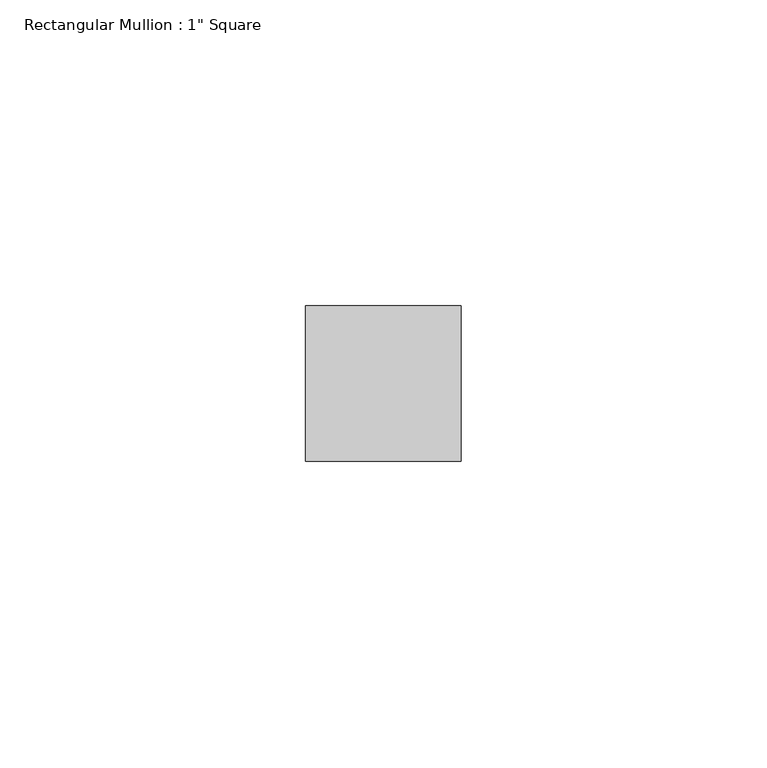
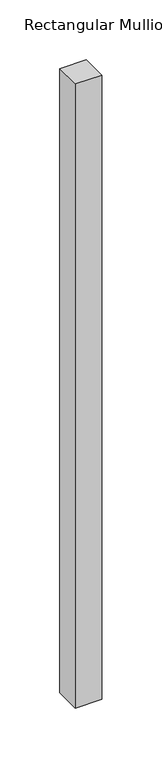
"""IFC4 building model written with IfcOpenShell, lengths in millimetres: member geometry."""

from ifc_helpers import new_model, si_unit, frame, origin, place, context, project, spatial, polyline, outline, extrude, source, transform, mapped, element, save


def member_795d39c7(model_context):
    return source(origin(), model_context, "Body", "SweptSolid", [
        extrude(outline(polyline([(12.7, 12.7), (12.7, -12.7), (-12.7, -12.7), (-12.7, 12.7), (12.7, 12.7)])), frame((0.0, 0.0, -635.0), z_axis=(0.0, 0.0, 1.0), x_axis=(1.0, 0.0, 0.0)), (0.0, 0.0, 1.0), 635.0),
    ])


if __name__ == "__main__":
    model = new_model("IFC4")
    model_context = context("Model", 3, world=origin())
    ifc_project = project(units=[si_unit("LENGTHUNIT", "METRE", prefix="MILLI")], contexts=[model_context])
    site = spatial("IfcSite", under=ifc_project)
    building = spatial("IfcBuilding", under=site)
    placement = place(None, origin())
    member_shape = member_795d39c7(model_context)
    element("IfcMember", 1, ObjectType="Rectangular Mullion : 1\" Square", at=placement, inside=building, context=model_context, shape_type="MappedRepresentation", body=[
        mapped(member_shape, transform((0.0, 0.0, 0.0), x_axis=(1.0, 0.0, 0.0), y_axis=(0.0, 1.0, 0.0), z_axis=(0.0, 0.0, 1.0))),
    ])
    save(model, "model.ifc")

# Revit data of these elements
# Type "Rectangular Mullion : 1\" Square"
#   built-in parameter 1007304 = 0.0833333 (stored number, unit not read)
#   built-in parameter 1007301 = 0.0416667 (stored number, unit not read)
#   built-in parameter 1007300 = 0.0416667 (stored number, unit not read)
# Element 1 (IfcMember, "Rectangular Mullion : 1\" Square")
#   Materials on its faces: "Metal - Aluminum"
# Materials
#   "Metal - Aluminum": class "Metal", colour RGB 247 247 247, transparency 0
